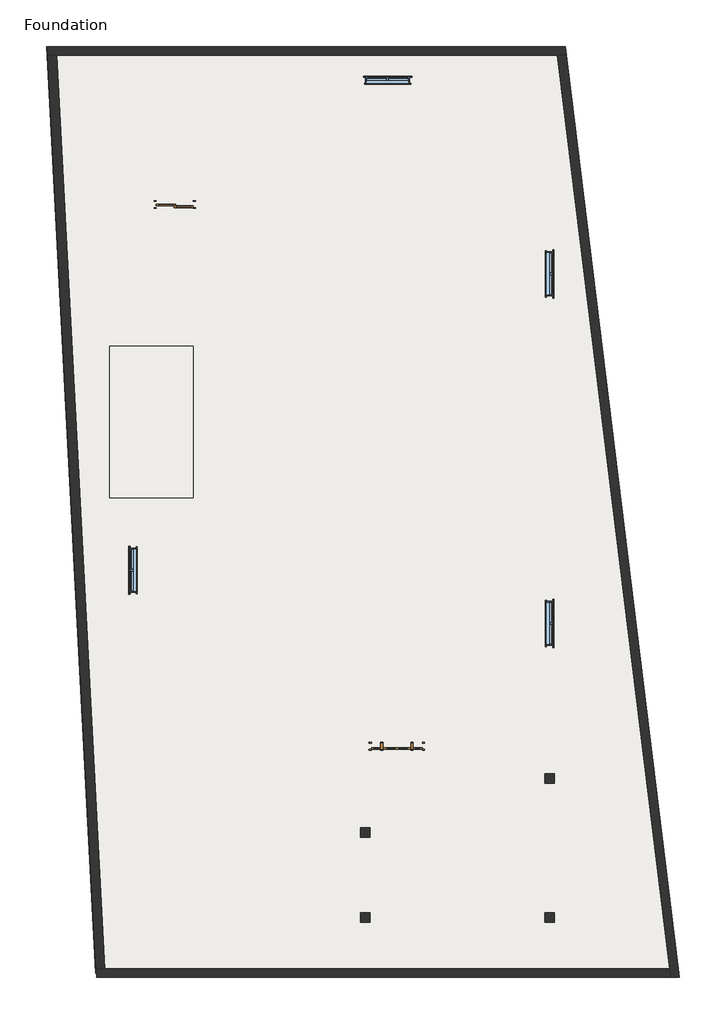
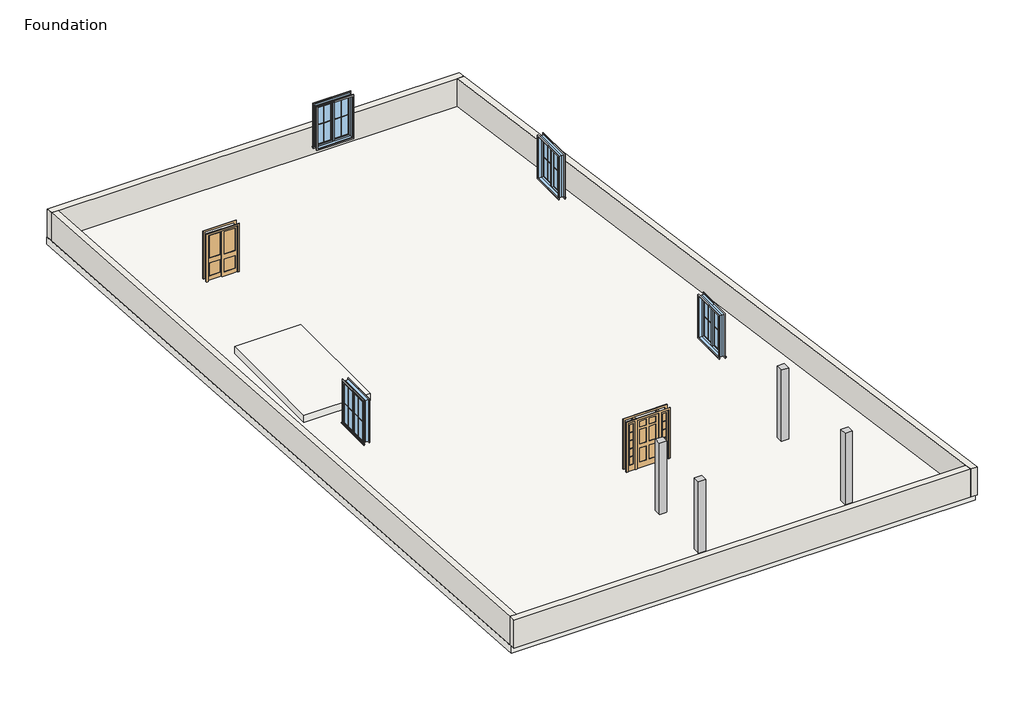
# One storey: 16 proxies, 4 columns, 4 walls, 4 windows, 2 doors, 2 slabs.
"""IFC4 building model written with IfcOpenShell, lengths in millimetres."""

import ifcopenshell
import ifcopenshell.guid

model = None  # the IFC model being written
_history = None  # IfcOwnerHistory: only IFC2X3 demands one
_inside = {}  # id of a spatial element -> (the spatial element, [elements in it])
_under = {}  # id of a project, library or spatial element -> (it, [spatial elements below it])
_declared = {}  # id of a project -> (the project, [libraries it declares])
_typed = {}  # id of a type object -> (the type object, [elements of that type])
_made_of = {}  # id of a material, layer set ... -> (it, [elements and type objects made of it])


def new_model(schema):
    """Start an empty IFC model of exactly this schema.

    Asked for "IFC4X3", IfcOpenShell would pick the latest addendum, in which some entities
    have other attributes; the version numbers below select the first issue.
    IFC2X3 requires an IfcOwnerHistory on every rooted entity: one is made here for all.
    """
    global model, _history
    if schema == "IFC4X3":
        model = ifcopenshell.file(schema_version=(4, 3, 0, 0))
    else:
        model = ifcopenshell.file(schema=schema)
    _inside.clear()
    _under.clear()
    _declared.clear()
    _typed.clear()
    _made_of.clear()
    _history = None
    if model.schema == "IFC2X3":
        org = make("IfcOrganization", Name="unknown")
        user = make(
            "IfcPersonAndOrganization",
            ThePerson=make("IfcPerson", FamilyName="unknown"),
            TheOrganization=org,
        )
        app = make(
            "IfcApplication",
            ApplicationDeveloper=org,
            Version="unknown",
            ApplicationFullName="unknown",
            ApplicationIdentifier="unknown",
        )
        _history = make(
            "IfcOwnerHistory",
            OwningUser=user,
            OwningApplication=app,
            ChangeAction="ADDED",
            CreationDate=0,
        )
    return model


def make(cls, **values):
    """One entity of the class cls with the attributes given. An attribute that is None is left unset."""
    return model.create_entity(
        cls, **{name: value for name, value in values.items() if value is not None}
    )


def rooted(cls, **values):
    """An entity with a GlobalId (a new one), such as an element, a storey or a relation."""
    return make(cls, GlobalId=ifcopenshell.guid.new(), OwnerHistory=_history, **values)


def si_unit(unit_type, name, prefix=None):
    """IfcSIUnit, for example si_unit("LENGTHUNIT", "METRE", prefix="MILLI")."""
    return make("IfcSIUnit", UnitType=unit_type, Prefix=prefix, Name=name)


def assignment(units):
    """IfcUnitAssignment: the units of a project."""
    return None if units is None else make("IfcUnitAssignment", Units=units)


def point(xyz):
    """IfcCartesianPoint."""
    return None if xyz is None else make("IfcCartesianPoint", Coordinates=xyz)


def direction(xyz):
    """IfcDirection."""
    return None if xyz is None else make("IfcDirection", DirectionRatios=xyz)


def frame(location, z_axis=None, x_axis=None):
    """IfcAxis2Placement3D, a coordinate frame: its origin and axes. An axis left out is left unset."""
    return make(
        "IfcAxis2Placement3D",
        Location=point(location),
        Axis=direction(z_axis),
        RefDirection=direction(x_axis),
    )


def origin():
    """The frame at (0, 0, 0) with its axes left unset."""
    return frame((0.0, 0.0, 0.0))


def origin_with_axes():
    """The frame at (0, 0, 0) with the z axis (0, 0, 1) and the x axis (1, 0, 0) written out."""
    return frame((0.0, 0.0, 0.0), z_axis=(0.0, 0.0, 1.0), x_axis=(1.0, 0.0, 0.0))


def place(relative_to, where):
    """IfcLocalPlacement: puts the frame where relative to a parent placement (None: the world)."""
    return make(
        "IfcLocalPlacement", PlacementRelTo=relative_to, RelativePlacement=where
    )


def context(
    kind, dimensions, precision=None, world=None, true_north=None, identifier=None
):
    """IfcGeometricRepresentationContext, for example the 3D "Model" context."""
    return make(
        "IfcGeometricRepresentationContext",
        ContextIdentifier=identifier,
        ContextType=kind,
        CoordinateSpaceDimension=dimensions,
        Precision=precision,
        WorldCoordinateSystem=world,
        TrueNorth=true_north,
    )


def project(units=None, contexts=None):
    """IfcProject with its units and contexts."""
    return rooted(
        "IfcProject",
        Name="project",
        RepresentationContexts=contexts,
        UnitsInContext=assignment(units),
    )


def spatial(cls, under=None, at=None, **own):
    """A site, building, storey or space (cls), placed at a placement, below another one or the project."""
    s = rooted(cls, ObjectPlacement=at, **own)
    if under is not None:
        _under.setdefault(under.id(), (under, []))[1].append(s)
    return s


def polyline(points):
    """IfcPolyline through the points."""
    return make("IfcPolyline", Points=[point(p) for p in points])


def outline(outer, holes=None, kind="AREA"):
    """IfcArbitraryClosedProfileDef: a profile drawn as a closed curve; with holes, ...WithVoids."""
    if holes is None:
        return make("IfcArbitraryClosedProfileDef", ProfileType=kind, OuterCurve=outer)
    return make(
        "IfcArbitraryProfileDefWithVoids",
        ProfileType=kind,
        OuterCurve=outer,
        InnerCurves=holes,
    )


def extrude(swept, where, along, depth):
    """IfcExtrudedAreaSolid: the profile swept, set in the frame where, extruded along a direction by depth."""
    return make(
        "IfcExtrudedAreaSolid",
        SweptArea=swept,
        Position=where,
        ExtrudedDirection=direction(along),
        Depth=depth,
    )


def faces_of(points, faces, orient=None, outer=None):
    """IfcFace entities. A face is a list of loops; a loop is a list of indices into points, from 0.

    orient and outer hold one flag for each loop. By default every Orientation is true, the
    first loop of a face is its IfcFaceOuterBound and the others are IfcFaceBound.
    """
    made = []
    for i, loops in enumerate(faces):
        bounds = []
        for j, loop in enumerate(loops):
            is_outer = j == 0 if outer is None else outer[i][j]
            bounds.append(
                make(
                    "IfcFaceOuterBound" if is_outer else "IfcFaceBound",
                    Bound=make("IfcPolyLoop", Polygon=[points[k] for k in loop]),
                    Orientation=True if orient is None else orient[i][j],
                )
            )
        made.append(make("IfcFace", Bounds=bounds))
    return made


def faceted_brep(points, faces, orient=None, outer=None, voids=None):
    """IfcFacetedBrep: a solid bounded by flat faces; with voids (closed shells), ...WithVoids."""
    shared = [point(p) for p in points]
    hull = make("IfcClosedShell", CfsFaces=faces_of(shared, faces, orient, outer))
    if voids is None:
        return make("IfcFacetedBrep", Outer=hull)
    return make(
        "IfcFacetedBrepWithVoids",
        Outer=hull,
        Voids=[
            make(cls, CfsFaces=faces_of(shared, fs, o, b)) for cls, fs, o, b in voids
        ],
    )


def shape(context_of_items, identifier, shape_type, items):
    """IfcShapeRepresentation: the items that make up one representation, for example the "Body"."""
    return make(
        "IfcShapeRepresentation",
        ContextOfItems=context_of_items,
        RepresentationIdentifier=identifier,
        RepresentationType=shape_type,
        Items=items,
    )


def source(mapping_origin, context_of_items, identifier, shape_type, items):
    """IfcRepresentationMap: a shape defined once, which mapped items show again and again."""
    return make(
        "IfcRepresentationMap",
        MappingOrigin=mapping_origin,
        MappedRepresentation=shape(context_of_items, identifier, shape_type, items),
    )


def transform(
    local_origin,
    x_axis=None,
    y_axis=None,
    z_axis=None,
    scale=None,
    scale2=None,
    scale3=None,
    uniform=True,
):
    """IfcCartesianTransformationOperator3D, or its non-uniform kind. x_axis, y_axis, z_axis: its Axis1, 2, 3."""
    if uniform:
        return make(
            "IfcCartesianTransformationOperator3D",
            Axis1=direction(x_axis),
            Axis2=direction(y_axis),
            LocalOrigin=point(local_origin),
            Scale=scale,
            Axis3=direction(z_axis),
        )
    return make(
        "IfcCartesianTransformationOperator3DnonUniform",
        Axis1=direction(x_axis),
        Axis2=direction(y_axis),
        LocalOrigin=point(local_origin),
        Scale=scale,
        Axis3=direction(z_axis),
        Scale2=scale2,
        Scale3=scale3,
    )


def mapped(mapping_source, mapping_target):
    """IfcMappedItem: shows the shape of a source again, moved by a transform."""
    return make(
        "IfcMappedItem", MappingSource=mapping_source, MappingTarget=mapping_target
    )


def made_of(thing, what):
    """Note that an element or type object is made of a material, layer set ...; save() writes the relation."""
    if what is not None:
        _made_of.setdefault(what.id(), (what, []))[1].append(thing)
    return thing


def element(
    cls,
    number,
    at=None,
    inside=None,
    cuts=None,
    type_object=None,
    material=None,
    context=None,
    identifier="Body",
    shape_type=None,
    held_by="IfcProductDefinitionShape",
    body=None,
    shapes=None,
    **own,
):
    """One element of the class cls, such as IfcWall. Its Tag is "e" and its number.

    at: its placement. inside: the storey or other place that contains it. cuts: it is an
    opening in that element (IfcRelVoidsElement). A single representation is given by context,
    identifier, shape_type and body (its items); several are given by shapes. held_by: the class
    of the entity that holds the representations. save() writes the other relations.
    """
    e = rooted(cls, Tag="e%d" % number, ObjectPlacement=at, **own)
    if body is not None:
        shapes = [shape(context, identifier, shape_type, body)]
    if shapes is not None:
        e.Representation = make(held_by, Representations=shapes)
    if inside is not None:
        _inside.setdefault(inside.id(), (inside, []))[1].append(e)
    if cuts is not None:
        rooted(
            "IfcRelVoidsElement", RelatingBuildingElement=cuts, RelatedOpeningElement=e
        )
    if type_object is not None:
        _typed.setdefault(type_object.id(), (type_object, []))[1].append(e)
    return made_of(e, material)


def aggregate(whole, parts):
    """IfcRelAggregates: a whole, such as a stair, and the parts it consists of."""
    return rooted("IfcRelAggregates", RelatingObject=whole, RelatedObjects=parts)


def save(model, path):
    """Write the relations noted so far, then the file.

    IfcRelAggregates (storeys below a building ...), IfcRelContainedInSpatialStructure (elements
    in a storey), IfcRelDefinesByType, IfcRelAssociatesMaterial and IfcRelDeclares: one each for
    every whole, place, type object, material and project.
    """
    for whole, parts in _under.values():
        aggregate(whole, parts)
    for where, things in _inside.values():
        rooted(
            "IfcRelContainedInSpatialStructure",
            RelatedElements=things,
            RelatingStructure=where,
        )
    for kind, things in _typed.values():
        rooted("IfcRelDefinesByType", RelatedObjects=things, RelatingType=kind)
    for what, things in _made_of.values():
        rooted("IfcRelAssociatesMaterial", RelatedObjects=things, RelatingMaterial=what)
    for by, libraries in _declared.values():
        rooted("IfcRelDeclares", RelatingContext=by, RelatedDefinitions=libraries)
    model.write(path)


def muntin_pattern_2x2_muntin_pattern_2x2_bff912c5(model_context):
    return source(origin(), model_context, "Body", "SweptSolid", [
        extrude(outline(polyline([(850.9, -6.35), (850.9, -293.6875), (838.2, -293.6875), (838.2, -6.35), (0.0, -6.35), (0.0, 6.35), (838.2, 6.35), (838.2, 293.6875), (850.9, 293.6875), (850.9, 6.35), (1689.1, 6.35), (1689.1, -6.35), (850.9, -6.35)])), frame((0.0, 9.525, 0.0), z_axis=(0.0, 1.0, 0.0), x_axis=(0.0, 0.0, 1.0)), (0.0, 0.0, 1.0), 12.7),
        extrude(outline(polyline([(850.9, -6.35), (850.9, -293.6875), (838.2, -293.6875), (838.2, -6.35), (0.0, -6.35), (0.0, 6.35), (838.2, 6.35), (838.2, 293.6875), (850.9, 293.6875), (850.9, 6.35), (1689.1, 6.35), (1689.1, -6.35), (850.9, -6.35)])), frame((0.0, -22.225, 0.0), z_axis=(0.0, 1.0, 0.0), x_axis=(0.0, 0.0, 1.0)), (0.0, 0.0, 1.0), 12.7),
    ])


def muntin_pattern_2x2_muntin_pattern_2x2_c2194282(model_context):
    return source(origin(), model_context, "Body", "SweptSolid", [
        extrude(outline(polyline([(850.9, -6.35), (850.9, -293.6875), (838.2, -293.6875), (838.2, -6.35), (0.0, -6.35), (0.0, 6.35), (838.2, 6.35), (838.2, 293.6875), (850.9, 293.6875), (850.9, 6.35), (1689.1, 6.35), (1689.1, -6.35), (850.9, -6.35)])), frame((0.0, -22.225, 0.0), z_axis=(0.0, 1.0, 0.0), x_axis=(0.0, 0.0, 1.0)), (0.0, 0.0, 1.0), 12.7),
        extrude(outline(polyline([(850.9, -6.35), (850.9, -293.6875), (838.2, -293.6875), (838.2, -6.35), (0.0, -6.35), (0.0, 6.35), (838.2, 6.35), (838.2, 293.6875), (850.9, 293.6875), (850.9, 6.35), (1689.1, 6.35), (1689.1, -6.35), (850.9, -6.35)])), frame((0.0, 9.525, 0.0), z_axis=(0.0, 1.0, 0.0), x_axis=(0.0, 0.0, 1.0)), (0.0, 0.0, 1.0), 12.7),
    ])


def trim_window_exterior_flat_with_sill_e04b3088(model_context):
    return source(origin(), model_context, "Body", "SweptSolid", [
        extrude(outline(polyline([(781.05, -1850.9823709), (781.05, -1908.1323709), (-781.05, -1908.1323709), (-781.05, -1850.9823709), (781.05, -1850.9823709)])), origin_with_axes(), (0.0, 0.0, 1.0), 19.05),
        extrude(outline(polyline([(-1860.55, 38.1), (-1831.2580645, 38.1), (-1828.8, 19.05), (-1828.8, 0.0), (-1850.9823709, 0.0), (-1850.9823709, 19.05), (-1860.55, 19.05), (-1860.55, 38.1)])), frame((-793.75, 0.0, 0.0), z_axis=(1.0, 0.0, 0.0), x_axis=(0.0, 1.0, 0.0)), (0.0, 0.0, 1.0), 1587.5),
        extrude(outline(polyline([(-781.05, 57.15), (781.05, 57.15), (781.05, -1828.8), (723.9, -1828.8), (723.9, 0.0), (-723.9, 0.0), (-723.9, -1828.8), (-781.05, -1828.8), (-781.05, 57.15)])), origin_with_axes(), (0.0, 0.0, 1.0), 19.05),
    ])


def trim_window_interior_flat_picture_frame_2a7685fe(model_context):
    return source(origin(), model_context, "Body", "SweptSolid", [
        extrude(outline(polyline([(768.35, 44.45), (768.35, -1873.25), (-768.35, -1873.25), (-768.35, 44.45), (768.35, 44.45)]), holes=[polyline([(711.2, -12.7), (-711.2, -12.7), (-711.2, -1816.1), (711.2, -1816.1), (711.2, -12.7)])]), origin_with_axes(), (0.0, 0.0, 1.0), 31.75),
    ])


def column_96c5ed10(model_context):
    return source(origin(), model_context, "Body", "SweptSolid", [
        extrude(outline(polyline([(152.4, 152.4), (152.4, -152.4), (-152.4, -152.4), (-152.4, 152.4), (152.4, 152.4)])), frame((0.0, 0.0, -381.0), z_axis=(0.0, 0.0, 1.0), x_axis=(1.0, 0.0, 0.0)), (0.0, 0.0, 1.0), 3124.2),
    ])


def door_4cad2e7a(model_context):
    return source(origin(), model_context, "Body", "SweptSolid", [
        extrude(outline(polyline([(762.0, 60.325), (609.6, 60.325), (609.6, 92.075), (762.0, 92.075), (762.0, 60.325)])), frame((0.0, 0.0, 600.075), z_axis=(0.0, 0.0, 1.0), x_axis=(1.0, 0.0, 0.0)), (0.0, 0.0, 1.0), 19.05),
        extrude(outline(polyline([(762.0, 60.325), (609.6, 60.325), (609.6, 92.075), (762.0, 92.075), (762.0, 60.325)])), frame((0.0, 0.0, 955.675), z_axis=(0.0, 0.0, 1.0), x_axis=(1.0, 0.0, 0.0)), (0.0, 0.0, 1.0), 19.05),
        extrude(outline(polyline([(762.0, 60.325), (609.6, 60.325), (609.6, 92.075), (762.0, 92.075), (762.0, 60.325)])), frame((0.0, 0.0, 1311.275), z_axis=(0.0, 0.0, 1.0), x_axis=(1.0, 0.0, 0.0)), (0.0, 0.0, 1.0), 19.05),
        extrude(outline(polyline([(762.0, 60.325), (609.6, 60.325), (609.6, 92.075), (762.0, 92.075), (762.0, 60.325)])), frame((0.0, 0.0, 1666.875), z_axis=(0.0, 0.0, 1.0), x_axis=(1.0, 0.0, 0.0)), (0.0, 0.0, 1.0), 19.05),
        extrude(outline(polyline([(-609.6, 60.325), (-762.0, 60.325), (-762.0, 92.075), (-609.6, 92.075), (-609.6, 60.325)])), frame((0.0, 0.0, 1666.875), z_axis=(0.0, 0.0, 1.0), x_axis=(1.0, 0.0, 0.0)), (0.0, 0.0, 1.0), 19.05),
        extrude(outline(polyline([(-609.6, 60.325), (-762.0, 60.325), (-762.0, 92.075), (-609.6, 92.075), (-609.6, 60.325)])), frame((0.0, 0.0, 1311.275), z_axis=(0.0, 0.0, 1.0), x_axis=(1.0, 0.0, 0.0)), (0.0, 0.0, 1.0), 19.05),
        extrude(outline(polyline([(-609.6, 60.325), (-762.0, 60.325), (-762.0, 92.075), (-609.6, 92.075), (-609.6, 60.325)])), frame((0.0, 0.0, 955.675), z_axis=(0.0, 0.0, 1.0), x_axis=(1.0, 0.0, 0.0)), (0.0, 0.0, 1.0), 19.05),
        extrude(outline(polyline([(-609.6, 60.325), (-762.0, 60.325), (-762.0, 92.075), (-609.6, 92.075), (-609.6, 60.325)])), frame((0.0, 0.0, 600.075), z_axis=(0.0, 0.0, 1.0), x_axis=(1.0, 0.0, 0.0)), (0.0, 0.0, 1.0), 19.05),
        extrude(outline(polyline([(762.0, 66.675), (609.6, 66.675), (609.6, 85.725), (762.0, 85.725), (762.0, 66.675)])), frame((0.0, 0.0, 254.0), z_axis=(0.0, 0.0, 1.0), x_axis=(1.0, 0.0, 0.0)), (0.0, 0.0, 1.0), 1778.0),
        extrude(outline(polyline([(-609.6, 66.675), (-762.0, 66.675), (-762.0, 85.725), (-609.6, 85.725), (-609.6, 66.675)])), frame((0.0, 0.0, 254.0), z_axis=(0.0, 0.0, 1.0), x_axis=(1.0, 0.0, 0.0)), (0.0, 0.0, 1.0), 1778.0),
        extrude(outline(polyline([(-457.2, -101.6), (-533.4, -101.6), (-533.4, 101.6), (-457.2, 101.6), (-457.2, -101.6)])), origin_with_axes(), (0.0, 0.0, 1.0), 2133.6),
        extrude(outline(polyline([(533.4, -101.6), (457.2, -101.6), (457.2, 101.6), (533.4, 101.6), (533.4, -101.6)])), origin_with_axes(), (0.0, 0.0, 1.0), 2133.6),
        extrude(outline(polyline([(2133.6, -533.4), (2133.6, -838.2), (0.0, -838.2), (0.0, -533.4), (2133.6, -533.4)]), holes=[polyline([(2032.0, -609.6), (254.0, -609.6), (254.0, -762.0), (2032.0, -762.0), (2032.0, -609.6)])]), frame((0.0, 50.8, 0.0), z_axis=(0.0, 1.0, 0.0), x_axis=(0.0, 0.0, 1.0)), (0.0, 0.0, 1.0), 50.8),
        extrude(outline(polyline([(0.0, 533.4), (0.0, 838.2), (2133.6, 838.2), (2133.6, 533.4), (0.0, 533.4)]), holes=[polyline([(2032.0, 762.0), (254.0, 762.0), (254.0, 609.6), (2032.0, 609.6), (2032.0, 762.0)])]), frame((0.0, 50.8, 0.0), z_axis=(0.0, 1.0, 0.0), x_axis=(0.0, 0.0, 1.0)), (0.0, 0.0, 1.0), 50.8),
        extrude(outline(polyline([(0.0, -914.4), (0.0, -838.2), (2133.6, -838.2), (2133.6, -533.4), (0.0, -533.4), (0.0, -457.2), (2133.6, -457.2), (2133.6, 457.2), (0.0, 457.2), (0.0, 533.4), (2133.6, 533.4), (2133.6, 838.2), (0.0, 838.2), (0.0, 914.4), (2209.8, 914.4), (2209.8, -914.4), (0.0, -914.4)])), frame((0.0, -127.0, 0.0), z_axis=(0.0, 1.0, 0.0), x_axis=(0.0, 0.0, 1.0)), (0.0, 0.0, 1.0), 25.4),
        extrude(outline(polyline([(0.0, 914.4), (2209.8, 914.4), (2209.8, -914.4), (0.0, -914.4), (0.0, -838.2), (2133.6, -838.2), (2133.6, -533.4), (0.0, -533.4), (0.0, -457.2), (2133.6, -457.2), (2133.6, 457.2), (0.0, 457.2), (0.0, 533.4), (2133.6, 533.4), (2133.6, 838.2), (0.0, 838.2), (0.0, 914.4)])), frame((0.0, 101.6, 0.0), z_axis=(0.0, 1.0, 0.0), x_axis=(0.0, 0.0, 1.0)), (0.0, 0.0, 1.0), 25.4),
        extrude(outline(polyline([(-63.5, 63.5), (-330.2, 63.5), (-330.2, 88.9), (-63.5, 88.9), (-63.5, 63.5)])), frame((0.0, 0.0, 1778.0), z_axis=(0.0, 0.0, 1.0), x_axis=(1.0, 0.0, 0.0)), (0.0, 0.0, 1.0), 254.0),
        extrude(outline(polyline([(330.2, 63.5), (63.5, 63.5), (63.5, 88.9), (330.2, 88.9), (330.2, 63.5)])), frame((0.0, 0.0, 1778.0), z_axis=(0.0, 0.0, 1.0), x_axis=(1.0, 0.0, 0.0)), (0.0, 0.0, 1.0), 254.0),
        extrude(outline(polyline([(-63.5, 63.5), (-330.2, 63.5), (-330.2, 88.9), (-63.5, 88.9), (-63.5, 63.5)])), frame((0.0, 0.0, 1041.4), z_axis=(0.0, 0.0, 1.0), x_axis=(1.0, 0.0, 0.0)), (0.0, 0.0, 1.0), 635.0),
        extrude(outline(polyline([(330.2, 63.5), (63.5, 63.5), (63.5, 88.9), (330.2, 88.9), (330.2, 63.5)])), frame((0.0, 0.0, 1041.4), z_axis=(0.0, 0.0, 1.0), x_axis=(1.0, 0.0, 0.0)), (0.0, 0.0, 1.0), 635.0),
        extrude(outline(polyline([(-63.5, 63.5), (-330.2, 63.5), (-330.2, 88.9), (-63.5, 88.9), (-63.5, 63.5)])), frame((0.0, 0.0, 254.0), z_axis=(0.0, 0.0, 1.0), x_axis=(1.0, 0.0, 0.0)), (0.0, 0.0, 1.0), 609.6),
        extrude(outline(polyline([(330.2, 63.5), (63.5, 63.5), (63.5, 88.9), (330.2, 88.9), (330.2, 63.5)])), frame((0.0, 0.0, 254.0), z_axis=(0.0, 0.0, 1.0), x_axis=(1.0, 0.0, 0.0)), (0.0, 0.0, 1.0), 609.6),
        extrude(outline(polyline([(2133.6, 457.2), (2133.6, -457.2), (0.0, -457.2), (0.0, 457.2), (2133.6, 457.2)]), holes=[polyline([(2032.0, -63.5), (1778.0, -63.5), (1778.0, -330.2), (2032.0, -330.2), (2032.0, -63.5)]), polyline([(2032.0, 330.2), (1778.0, 330.2), (1778.0, 63.5), (2032.0, 63.5), (2032.0, 330.2)]), polyline([(1676.4, -63.5), (1041.4, -63.5), (1041.4, -330.2), (1676.4, -330.2), (1676.4, -63.5)]), polyline([(1676.4, 330.2), (1041.4, 330.2), (1041.4, 63.5), (1676.4, 63.5), (1676.4, 330.2)]), polyline([(863.6, -63.5), (254.0, -63.5), (254.0, -330.2), (863.6, -330.2), (863.6, -63.5)]), polyline([(863.6, 330.2), (254.0, 330.2), (254.0, 63.5), (863.6, 63.5), (863.6, 330.2)])]), frame((0.0, 50.8, 0.0), z_axis=(0.0, 1.0, 0.0), x_axis=(0.0, 0.0, 1.0)), (0.0, 0.0, 1.0), 50.8),
    ])


def door_5d877b8f(model_context):
    return source(origin(), model_context, "Body", "SweptSolid", [
        extrude(outline(polyline([(-63.5, 190.5), (-520.7, 190.5), (-520.7, 215.9), (-63.5, 215.9), (-63.5, 190.5)])), frame((0.0, 0.0, 965.2), z_axis=(0.0, 0.0, 1.0), x_axis=(1.0, 0.0, 0.0)), (0.0, 0.0, 1.0), 977.9),
        extrude(outline(polyline([(-63.5, 190.5), (-520.7, 190.5), (-520.7, 215.9), (-63.5, 215.9), (-63.5, 190.5)])), frame((0.0, 0.0, 184.15), z_axis=(0.0, 0.0, 1.0), x_axis=(1.0, 0.0, 0.0)), (0.0, 0.0, 1.0), 565.15),
        extrude(outline(polyline([(63.5, 165.1), (520.7, 165.1), (520.7, 139.7), (63.5, 139.7), (63.5, 165.1)])), frame((0.0, 0.0, 965.2), z_axis=(0.0, 0.0, 1.0), x_axis=(1.0, 0.0, 0.0)), (0.0, 0.0, 1.0), 977.9),
        extrude(outline(polyline([(63.5, 165.1), (520.7, 165.1), (520.7, 139.7), (63.5, 139.7), (63.5, 165.1)])), frame((0.0, 0.0, 184.15), z_axis=(0.0, 0.0, 1.0), x_axis=(1.0, 0.0, 0.0)), (0.0, 0.0, 1.0), 565.15),
        extrude(outline(polyline([(2032.0, 25.4), (2032.0, -609.6), (0.0, -609.6), (0.0, 25.4), (2032.0, 25.4)]), holes=[polyline([(184.15, -520.7), (749.3, -520.7), (749.3, -63.5), (184.15, -63.5), (184.15, -520.7)]), polyline([(965.2, -520.7), (1943.1, -520.7), (1943.1, -63.5), (965.2, -63.5), (965.2, -520.7)])]), frame((0.0, 177.8, 0.0), z_axis=(0.0, 1.0, 0.0), x_axis=(0.0, 0.0, 1.0)), (0.0, 0.0, 1.0), 50.8),
        extrude(outline(polyline([(0.0, -685.8), (0.0, -609.6), (2032.0, -609.6), (2032.0, 609.6), (0.0, 609.6), (0.0, 685.8), (2108.2, 685.8), (2108.2, -685.8), (0.0, -685.8)])), frame((0.0, 0.0, 0.0), z_axis=(0.0, 1.0, 0.0), x_axis=(0.0, 0.0, 1.0)), (0.0, 0.0, 1.0), 25.4),
        extrude(outline(polyline([(0.0, 685.8), (2108.2, 685.8), (2108.2, -685.8), (0.0, -685.8), (0.0, -609.6), (2032.0, -609.6), (2032.0, 609.6), (0.0, 609.6), (0.0, 685.8)])), frame((0.0, 228.6, 0.0), z_axis=(0.0, 1.0, 0.0), x_axis=(0.0, 0.0, 1.0)), (0.0, 0.0, 1.0), 25.4),
        extrude(outline(polyline([(2032.0, -25.4), (0.0, -25.4), (0.0, 609.6), (2032.0, 609.6), (2032.0, -25.4)]), holes=[polyline([(965.2, 520.7), (965.2, 63.5), (1943.1, 63.5), (1943.1, 520.7), (965.2, 520.7)]), polyline([(184.15, 520.7), (184.15, 63.5), (749.3, 63.5), (749.3, 520.7), (184.15, 520.7)])]), frame((0.0, 127.0, 0.0), z_axis=(0.0, 1.0, 0.0), x_axis=(0.0, 0.0, 1.0)), (0.0, 0.0, 1.0), 50.8),
    ])


def window_c580ef63(model_context):
    return source(origin(), model_context, "Body", "SolidModel", [
        faceted_brep([(9.525, 120.65, 2730.5), (-9.525, 120.65, 2730.5), (-9.525, 69.85, 2730.5), (9.525, 69.85, 2730.5), (9.525, 120.65, 927.1), (9.525, 69.85, 927.1), (-9.525, 69.85, 927.1), (-9.525, 120.65, 927.1), (-9.525, 69.85, 946.15), (-9.525, 69.85, 2711.45), (-30.1625, 69.85, 946.15), (-30.1625, 69.85, 2711.45), (-30.1625, 6.35, 946.15), (-30.1625, 6.35, 2711.45), (30.1625, 6.35, 946.15), (30.1625, 6.35, 2711.45), (30.1625, 69.85, 946.15), (30.1625, 69.85, 2711.45), (9.525, 69.85, 946.15), (9.525, 69.85, 2711.45)], [[[0, 1, 2, 3]], [[4, 5, 6, 7]], [[1, 0, 4, 7]], [[2, 1, 7, 6, 8, 9]], [[9, 8, 10, 11]], [[11, 10, 12, 13]], [[13, 12, 14, 15]], [[15, 14, 16, 17]], [[17, 16, 18, 19]], [[0, 3, 19, 18, 5, 4]], [[18, 8, 6, 5]], [[9, 19, 3, 2]], [[8, 18, 16, 14, 12, 10]], [[19, 9, 11, 13, 15, 17]]]),
        extrude(outline(polyline([(-66.675, 101.6), (-66.675, 95.25), (-654.05, 95.25), (-654.05, 101.6), (-66.675, 101.6)])), frame((0.0, 0.0, 984.25), z_axis=(0.0, 0.0, 1.0), x_axis=(1.0, 0.0, 0.0)), (0.0, 0.0, 1.0), 1689.1),
        extrude(outline(polyline([(-654.05, 82.55), (-654.05, 88.9), (-66.675, 88.9), (-66.675, 82.55), (-654.05, 82.55)])), frame((0.0, 0.0, 984.25), z_axis=(0.0, 0.0, 1.0), x_axis=(1.0, 0.0, 0.0)), (0.0, 0.0, 1.0), 1689.1),
        extrude(outline(polyline([(654.05, 101.6), (654.05, 95.25), (66.675, 95.25), (66.675, 101.6), (654.05, 101.6)])), frame((0.0, 0.0, 984.25), z_axis=(0.0, 0.0, 1.0), x_axis=(1.0, 0.0, 0.0)), (0.0, 0.0, 1.0), 1689.1),
        extrude(outline(polyline([(66.675, 82.55), (66.675, 88.9), (654.05, 88.9), (654.05, 82.55), (66.675, 82.55)])), frame((0.0, 0.0, 984.25), z_axis=(0.0, 0.0, 1.0), x_axis=(1.0, 0.0, 0.0)), (0.0, 0.0, 1.0), 1689.1),
        extrude(outline(polyline([(2730.5, -711.2), (927.1, -711.2), (927.1, -9.525), (2730.5, -9.525), (2730.5, -711.2)]), holes=[polyline([(2673.35, -66.675), (984.25, -66.675), (984.25, -654.05), (2673.35, -654.05), (2673.35, -66.675)])]), frame((0.0, 69.85, 0.0), z_axis=(0.0, 1.0, 0.0), x_axis=(0.0, 0.0, 1.0)), (0.0, 0.0, 1.0), 44.45),
        extrude(outline(polyline([(927.1, 711.2), (2730.5, 711.2), (2730.5, 9.525), (927.1, 9.525), (927.1, 711.2)]), holes=[polyline([(984.25, 66.675), (2673.35, 66.675), (2673.35, 654.05), (984.25, 654.05), (984.25, 66.675)])]), frame((0.0, 69.85, 0.0), z_axis=(0.0, 1.0, 0.0), x_axis=(0.0, 0.0, 1.0)), (0.0, 0.0, 1.0), 44.45),
        extrude(outline(polyline([(2743.2, -723.9), (914.4, -723.9), (914.4, 723.9), (2743.2, 723.9), (2743.2, -723.9)]), holes=[polyline([(2724.15, 704.85), (933.45, 704.85), (933.45, -704.85), (2724.15, -704.85), (2724.15, 704.85)])]), frame((0.0, -101.6, 0.0), z_axis=(0.0, 1.0, 0.0), x_axis=(0.0, 0.0, 1.0)), (0.0, 0.0, 1.0), 107.95),
        faceted_brep([(692.15, 69.85, 2711.45), (692.15, 6.35, 2711.45), (-692.15, 6.35, 2711.45), (-692.15, 69.85, 2711.45), (711.2, 120.65, 2730.5), (711.2, 69.85, 2730.5), (-711.2, 69.85, 2730.5), (-711.2, 120.65, 2730.5), (723.9, 6.35, 2743.2), (723.9, 120.65, 2743.2), (-723.9, 120.65, 2743.2), (-723.9, 6.35, 2743.2), (-692.15, 6.35, 946.15), (-692.15, 69.85, 946.15), (-711.2, 69.85, 927.1), (-711.2, 120.65, 927.1), (-723.9, 120.65, 914.4), (-723.9, 6.35, 914.4), (692.15, 6.35, 946.15), (692.15, 69.85, 946.15), (711.2, 69.85, 927.1), (711.2, 120.65, 927.1), (723.9, 120.65, 914.4), (723.9, 6.35, 914.4)], [[[0, 1, 2, 3]], [[4, 5, 6, 7]], [[8, 9, 10, 11]], [[3, 2, 12, 13]], [[7, 6, 14, 15]], [[11, 10, 16, 17]], [[13, 12, 18, 19]], [[15, 14, 20, 21]], [[17, 16, 22, 23]], [[11, 17, 23, 8], [1, 18, 12, 2]], [[19, 18, 1, 0]], [[5, 20, 14, 6], [3, 13, 19, 0]], [[21, 20, 5, 4]], [[23, 22, 9, 8]], [[9, 22, 16, 10], [7, 15, 21, 4]]]),
    ])


model = new_model("IFC4")

# Units and contexts
model_context = context("Model", 3, world=origin())
ifc_project = project(units=[si_unit("LENGTHUNIT", "METRE", prefix="MILLI")], contexts=[model_context])

# Site, building, storey
site = spatial("IfcSite", under=ifc_project)
building = spatial("IfcBuilding", under=site)
storey = spatial("IfcBuildingStorey", under=building, Name="Foundation", Elevation=-381.0)

# Proxies
placement = place(None, origin())
muntin_pattern_2x2_muntin_pattern_2x2_shape = muntin_pattern_2x2_muntin_pattern_2x2_bff912c5(model_context)
element("IfcBuildingElementProxy", 1, Name="Muntin Pattern_2x2 : Muntin Pattern_2x2", ObjectType="Muntin Pattern_2x2 : Muntin Pattern_2x2", at=placement, inside=storey, context=model_context, shape_type="MappedRepresentation", body=[
    mapped(muntin_pattern_2x2_muntin_pattern_2x2_shape, transform((-4271.6763913, -8364.6154211, 603.25), x_axis=(0.0, 1.0, 0.0), y_axis=(-1.0, 0.0, 0.0), z_axis=(0.0, 0.0, 1.0))),
])
element("IfcBuildingElementProxy", 2, Name="Muntin Pattern_2x2 : Muntin Pattern_2x2", ObjectType="Muntin Pattern_2x2 : Muntin Pattern_2x2", at=placement, inside=storey, context=model_context, shape_type="MappedRepresentation", body=[
    mapped(muntin_pattern_2x2_muntin_pattern_2x2_shape, transform((9628.4736087, -9396.4904211, 603.25), x_axis=(0.0, -1.0, 0.0), y_axis=(1.0, 0.0, 0.0), z_axis=(0.0, 0.0, 1.0))),
])
element("IfcBuildingElementProxy", 3, Name="Muntin Pattern_2x2 : Muntin Pattern_2x2", ObjectType="Muntin Pattern_2x2 : Muntin Pattern_2x2", at=placement, inside=storey, context=model_context, shape_type="MappedRepresentation", body=[
    mapped(muntin_pattern_2x2_muntin_pattern_2x2_shape, transform((9628.4736087, 2109.7095789, 603.25), x_axis=(0.0, -1.0, 0.0), y_axis=(1.0, 0.0, 0.0), z_axis=(0.0, 0.0, 1.0))),
])
element("IfcBuildingElementProxy", 4, Name="Muntin Pattern_2x2 : Muntin Pattern_2x2", ObjectType="Muntin Pattern_2x2 : Muntin Pattern_2x2", at=placement, inside=storey, context=model_context, shape_type="MappedRepresentation", body=[
    mapped(muntin_pattern_2x2_muntin_pattern_2x2_shape, transform((3842.0361087, 8211.5138811, 603.25), x_axis=(1.0, 0.0, 0.0), y_axis=(0.0, 1.0, 0.0), z_axis=(0.0, 0.0, 1.0))),
])
muntin_pattern_2x2_muntin_pattern_2x2_2_shape = muntin_pattern_2x2_muntin_pattern_2x2_c2194282(model_context)
element("IfcBuildingElementProxy", 5, Name="Muntin Pattern_2x2 : Muntin Pattern_2x2", ObjectType="Muntin Pattern_2x2 : Muntin Pattern_2x2", at=placement, inside=storey, context=model_context, shape_type="MappedRepresentation", body=[
    mapped(muntin_pattern_2x2_muntin_pattern_2x2_2_shape, transform((-4271.6763913, -7643.8904211, 603.25), x_axis=(0.0, -1.0, 0.0), y_axis=(1.0, 0.0, 0.0), z_axis=(0.0, 0.0, 1.0))),
])
element("IfcBuildingElementProxy", 6, Name="Muntin Pattern_2x2 : Muntin Pattern_2x2", ObjectType="Muntin Pattern_2x2 : Muntin Pattern_2x2", at=placement, inside=storey, context=model_context, shape_type="MappedRepresentation", body=[
    mapped(muntin_pattern_2x2_muntin_pattern_2x2_2_shape, transform((9628.4736087, -10117.2154211, 603.25), x_axis=(0.0, 1.0, 0.0), y_axis=(-1.0, 0.0, 0.0), z_axis=(0.0, 0.0, 1.0))),
])
element("IfcBuildingElementProxy", 7, Name="Muntin Pattern_2x2 : Muntin Pattern_2x2", ObjectType="Muntin Pattern_2x2 : Muntin Pattern_2x2", at=placement, inside=storey, context=model_context, shape_type="MappedRepresentation", body=[
    mapped(muntin_pattern_2x2_muntin_pattern_2x2_2_shape, transform((9628.4736087, 1388.9845789, 603.25), x_axis=(0.0, 1.0, 0.0), y_axis=(-1.0, 0.0, 0.0), z_axis=(0.0, 0.0, 1.0))),
])
element("IfcBuildingElementProxy", 8, Name="Muntin Pattern_2x2 : Muntin Pattern_2x2", ObjectType="Muntin Pattern_2x2 : Muntin Pattern_2x2", at=placement, inside=storey, context=model_context, shape_type="MappedRepresentation", body=[
    mapped(muntin_pattern_2x2_muntin_pattern_2x2_2_shape, transform((4562.7611087, 8211.5138811, 603.25), x_axis=(-1.0, 0.0, 0.0), y_axis=(0.0, -1.0, 0.0), z_axis=(0.0, 0.0, 1.0))),
])
trim_window_exterior_flat_with_sill_shape = trim_window_exterior_flat_with_sill_e04b3088(model_context)
element("IfcBuildingElementProxy", 9, Name="Trim-Window-Exterior-Flat : with Sill", ObjectType="Trim-Window-Exterior-Flat : with Sill", at=placement, inside=storey, context=model_context, shape_type="MappedRepresentation", body=[
    mapped(trim_window_exterior_flat_with_sill_shape, transform((-4281.2013913, -8004.2529211, 2362.2), x_axis=(0.0, -1.0, 0.0), y_axis=(0.0, 0.0, 1.0), z_axis=(-1.0, 0.0, 0.0))),
])
element("IfcBuildingElementProxy", 10, Name="Trim-Window-Exterior-Flat : with Sill", ObjectType="Trim-Window-Exterior-Flat : with Sill", at=placement, inside=storey, context=model_context, shape_type="MappedRepresentation", body=[
    mapped(trim_window_exterior_flat_with_sill_shape, transform((9637.9986087, -9756.8529211, 2362.2), x_axis=(0.0, 1.0, 0.0), y_axis=(0.0, 0.0, 1.0), z_axis=(1.0, 0.0, 0.0))),
])
element("IfcBuildingElementProxy", 11, Name="Trim-Window-Exterior-Flat : with Sill", ObjectType="Trim-Window-Exterior-Flat : with Sill", at=placement, inside=storey, context=model_context, shape_type="MappedRepresentation", body=[
    mapped(trim_window_exterior_flat_with_sill_shape, transform((9637.9986087, 1749.3470789, 2362.2), x_axis=(0.0, 1.0, 0.0), y_axis=(0.0, 0.0, 1.0), z_axis=(1.0, 0.0, 0.0))),
])
element("IfcBuildingElementProxy", 12, Name="Trim-Window-Exterior-Flat : with Sill", ObjectType="Trim-Window-Exterior-Flat : with Sill", at=placement, inside=storey, context=model_context, shape_type="MappedRepresentation", body=[
    mapped(trim_window_exterior_flat_with_sill_shape, transform((4202.3986087, 8221.0388811, 2362.2), x_axis=(-1.0, 0.0, 0.0), y_axis=(0.0, 0.0, 1.0), z_axis=(0.0, 1.0, 0.0))),
])
trim_window_interior_flat_picture_frame_shape = trim_window_interior_flat_picture_frame_2a7685fe(model_context)
element("IfcBuildingElementProxy", 13, Name="Trim-Window-Interior-Flat : Picture Frame", ObjectType="Trim-Window-Interior-Flat : Picture Frame", at=placement, inside=storey, context=model_context, shape_type="MappedRepresentation", body=[
    mapped(trim_window_interior_flat_picture_frame_shape, transform((-4078.0013913, -8004.2529211, 2362.2), x_axis=(0.0, 1.0, 0.0), y_axis=(0.0, 0.0, 1.0), z_axis=(1.0, 0.0, 0.0))),
])
element("IfcBuildingElementProxy", 14, Name="Trim-Window-Interior-Flat : Picture Frame", ObjectType="Trim-Window-Interior-Flat : Picture Frame", at=placement, inside=storey, context=model_context, shape_type="MappedRepresentation", body=[
    mapped(trim_window_interior_flat_picture_frame_shape, transform((9434.7986087, -9756.8529211, 2362.2), x_axis=(0.0, -1.0, 0.0), y_axis=(0.0, 0.0, 1.0), z_axis=(-1.0, 0.0, 0.0))),
])
element("IfcBuildingElementProxy", 15, Name="Trim-Window-Interior-Flat : Picture Frame", ObjectType="Trim-Window-Interior-Flat : Picture Frame", at=placement, inside=storey, context=model_context, shape_type="MappedRepresentation", body=[
    mapped(trim_window_interior_flat_picture_frame_shape, transform((9434.7986087, 1749.3470789, 2362.2), x_axis=(0.0, -1.0, 0.0), y_axis=(0.0, 0.0, 1.0), z_axis=(-1.0, 0.0, 0.0))),
])
element("IfcBuildingElementProxy", 16, Name="Trim-Window-Interior-Flat : Picture Frame", ObjectType="Trim-Window-Interior-Flat : Picture Frame", at=placement, inside=storey, context=model_context, shape_type="MappedRepresentation", body=[
    mapped(trim_window_interior_flat_picture_frame_shape, transform((4202.3986087, 8017.8388811, 2362.2), x_axis=(1.0, 0.0, 0.0), y_axis=(0.0, 0.0, 1.0), z_axis=(0.0, -1.0, 0.0))),
])

# Columns
column_shape = column_96c5ed10(model_context)
element("IfcColumn", 17, ObjectType="Rectangular Column : 12\" x 12\"", at=placement, inside=storey, context=model_context, shape_type="MappedRepresentation", body=[
    mapped(column_shape, transform((3465.7986087, -16640.2529211, 0.0), x_axis=(0.0, 1.0, 0.0), y_axis=(-1.0, 0.0, 0.0), z_axis=(0.0, 0.0, 1.0))),
])
element("IfcColumn", 18, ObjectType="Rectangular Column : 12\" x 12\"", at=placement, inside=storey, context=model_context, shape_type="MappedRepresentation", body=[
    mapped(column_shape, transform((9536.3986087, -14862.2529211, 0.0), x_axis=(0.0, 1.0, 0.0), y_axis=(-1.0, 0.0, 0.0), z_axis=(0.0, 0.0, 1.0))),
])
element("IfcColumn", 19, ObjectType="Rectangular Column : 12\" x 12\"", at=placement, inside=storey, context=model_context, shape_type="MappedRepresentation", body=[
    mapped(column_shape, transform((9536.3986087, -19434.2529211, 0.0), x_axis=(0.0, 1.0, 0.0), y_axis=(-1.0, 0.0, 0.0), z_axis=(0.0, 0.0, 1.0))),
])
element("IfcColumn", 20, ObjectType="Rectangular Column : 12\" x 12\"", at=placement, inside=storey, context=model_context, shape_type="MappedRepresentation", body=[
    mapped(column_shape, transform((3465.7986087, -19434.2529211, 0.0), x_axis=(0.0, 1.0, 0.0), y_axis=(-1.0, 0.0, 0.0), z_axis=(0.0, 0.0, 1.0))),
])

# Doors
door_shape = door_4cad2e7a(model_context)
element("IfcDoor", 21, ObjectType="Single-Raised Panel with Sidelights : 36\" x 84\"", at=placement, inside=storey, context=model_context, shape_type="MappedRepresentation", body=[
    mapped(door_shape, transform((4507.1986087, -13795.4529211, -381.0), x_axis=(-1.0, 0.0, 0.0), y_axis=(0.0, -1.0, 0.0), z_axis=(0.0, 0.0, 1.0))),
])
door_2_shape = door_5d877b8f(model_context)
element("IfcDoor", 22, ObjectType="Sliding-Closet : 48\" x 80\"", at=placement, inside=storey, context=model_context, shape_type="MappedRepresentation", body=[
    mapped(door_2_shape, transform((-2808.0013913, 4162.3470789, -381.0), x_axis=(-1.0, 0.0, 0.0), y_axis=(0.0, -1.0, 0.0), z_axis=(0.0, 0.0, 1.0))),
])

# Slabs
element("IfcSlab", 23, ObjectType="Concrete Slab - 12\" 2", at=placement, inside=storey, context=model_context, shape_type="SweptSolid", body=[
    extrude(outline(polyline([(10025.1414378, 9232.4757765), (13795.4376886, -21276.6158374), (-5406.9623114, -21276.6158374), (-7033.0961859, 9232.4757765), (10025.1414378, 9232.4757765)])), frame((0.0, 0.0, -685.8), z_axis=(0.0, 0.0, 1.0), x_axis=(1.0, 0.0, 0.0)), (0.0, 0.0, 1.0), 304.8),
])
element("IfcSlab", 24, ObjectType="Generic - 12\" Grass", at=placement, inside=storey, context=model_context, shape_type="SweptSolid", body=[
    extrude(outline(polyline([(-4949.7178966, -638.2529211), (-2206.5178966, -638.2529211), (-2206.5178966, -5616.6529211), (-4949.7178966, -5616.6529211), (-4949.7178966, -638.2529211)])), frame((0.0, 0.0, -228.6), z_axis=(0.0, 0.0, 1.0), x_axis=(1.0, 0.0, 0.0)), (0.0, 0.0, 1.0), 304.8),
])

# Walls
element("IfcWall", 25, ObjectType="Exterior - Brick on Wood Stud", at=placement, inside=storey, context=model_context, shape_type="Brep", body=[
    faceted_brep([(-6987.4030616, 8949.9007765, -381.0), (-6704.4321039, 8949.9007765, -381.0), (9799.3910296, 8949.9007765, -381.0), (10084.0881186, 8949.9007765, -381.0), (10084.0881186, 8949.9007765, 838.2), (9799.3910296, 8949.9007765, 838.2), (-6704.4321039, 8949.9007765, 838.2), (-6987.4030616, 8949.9007765, 838.2), (-7002.3674275, 9232.4757765, -381.0), (-7002.3674275, 9232.4757765, 838.2), (10049.3922713, 9232.4757765, 838.2), (10049.3922713, 9232.4757765, -381.0)], [[[0, 1, 2, 3, 4, 5, 6, 7]], [[8, 9, 10, 11]], [[3, 2, 1, 0, 8, 11]], [[7, 6, 5, 4, 10, 9]], [[4, 3, 11, 10]], [[0, 7, 9, 8]]]),
])
element("IfcWall", 26, ObjectType="Exterior - Brick on Wood Stud", at=placement, inside=storey, context=model_context, shape_type="Brep", body=[
    faceted_brep([(9799.3910296, 8949.9007765, -381.0), (13492.1677118, -21125.3518039, -381.0), (13526.8635591, -21407.9268039, -381.0), (13526.8635591, -21407.9268039, 838.2), (13492.1677118, -21125.3518039, 838.2), (9799.3910296, 8949.9007765, 838.2), (10084.0881186, 8949.9007765, -381.0), (10084.0881186, 8949.9007765, 838.2), (13811.560648, -21407.9268039, 838.2), (13811.560648, -21407.9268039, -381.0)], [[[0, 1, 2, 3, 4, 5]], [[6, 7, 8, 9]], [[2, 1, 0, 6, 9]], [[5, 4, 3, 8, 7]], [[0, 5, 7, 6]], [[3, 2, 9, 8]]]),
])
element("IfcWall", 27, ObjectType="Exterior - Brick on Wood Stud", at=placement, inside=storey, context=model_context, shape_type="Brep", body=[
    faceted_brep([(13492.1677118, -21125.3518039, -381.0), (-5111.7325242, -21125.3518039, -381.0), (-5394.7034819, -21125.3518039, -381.0), (-5394.7034819, -21125.3518039, 838.2), (-5111.7325242, -21125.3518039, 838.2), (13492.1677118, -21125.3518039, 838.2), (13526.8635591, -21407.9268039, -381.0), (13526.8635591, -21407.9268039, 838.2), (-5379.739116, -21407.9268039, 838.2), (-5379.739116, -21407.9268039, -381.0)], [[[0, 1, 2, 3, 4, 5]], [[6, 7, 8, 9]], [[2, 1, 0, 6, 9]], [[5, 4, 3, 8, 7]], [[0, 5, 7, 6]], [[3, 2, 9, 8]]]),
])
element("IfcWall", 28, ObjectType="Exterior - Brick on Wood Stud", at=placement, inside=storey, context=model_context, shape_type="SweptSolid", body=[
    extrude(outline(polyline([(-6704.4321039, 8949.9007765), (-5111.7325242, -21125.3518039), (-5394.7034819, -21125.3518039), (-6987.4030616, 8949.9007765), (-6704.4321039, 8949.9007765)])), frame((0.0, 0.0, -381.0), z_axis=(0.0, 0.0, 1.0), x_axis=(1.0, 0.0, 0.0)), (0.0, 0.0, 1.0), 1219.2),
])

# Windows
window_shape = window_c580ef63(model_context)
element("IfcWindow", 29, ObjectType="Window-Casement-Double : 57\" x 72\"", at=placement, inside=storey, context=model_context, shape_type="MappedRepresentation", body=[
    mapped(window_shape, transform((-4179.6013913, -8004.2529211, -381.0), x_axis=(0.0, 1.0, 0.0), y_axis=(-1.0, 0.0, 0.0), z_axis=(0.0, 0.0, 1.0))),
])
element("IfcWindow", 30, ObjectType="Window-Casement-Double : 57\" x 72\"", at=placement, inside=storey, context=model_context, shape_type="MappedRepresentation", body=[
    mapped(window_shape, transform((9536.3986087, -9756.8529211, -381.0), x_axis=(0.0, -1.0, 0.0), y_axis=(1.0, 0.0, 0.0), z_axis=(0.0, 0.0, 1.0))),
])
element("IfcWindow", 31, ObjectType="Window-Casement-Double : 57\" x 72\"", at=placement, inside=storey, context=model_context, shape_type="MappedRepresentation", body=[
    mapped(window_shape, transform((9536.3986087, 1749.3470789, -381.0), x_axis=(0.0, -1.0, 0.0), y_axis=(1.0, 0.0, 0.0), z_axis=(0.0, 0.0, 1.0))),
])
element("IfcWindow", 32, ObjectType="Window-Casement-Double : 57\" x 72\"", at=placement, inside=storey, context=model_context, shape_type="MappedRepresentation", body=[
    mapped(window_shape, transform((4202.3986087, 8119.4388811, -381.0), x_axis=(1.0, 0.0, 0.0), y_axis=(0.0, 1.0, 0.0), z_axis=(0.0, 0.0, 1.0))),
])

save(model, "model.ifc")

# Revit data of these elements
# Project information
#   Project Issue Date = "Issue Date"
#   Project Status = "Project Status"
#   Client Name = "Owner"
#   Project Address = "Enter address here"
#   Project Name = "Project Name"
#   Project Number = "Project Number"
# Type "Muntin Pattern_2x2 : Muntin Pattern_2x2"
#   Width [instance default] = 4' - 0"
#   Thickness = 0' - 0 1/2"
#   Height [instance default] = 4' - 0"
#   Distance = 0' - 0 3/4"
#   Interior Material [instance default] = none
#   Exterior Material [instance default] = none
#   Default Elevation = 0
# Type "Trim-Window-Exterior-Flat : with Sill"
#   Trim Width = 0' - 2 1/4"
#   Trim Thickness_Picture Frame = 0' - 1 1/4"
#   Trim Thickness_with Sill = 0' - 0 3/4"
#   Sill Thickness = 0' - 1 1/4"
#   Opening Width [instance default] = 2' - 0"
#   Opening Height [instance default] = 3' - 0"
#   Default Elevation = 4' - 0"
#   Sill = yes
#   Picture Frame = no
#   Trim Material [instance default] = none
# Type "Trim-Window-Interior-Flat : Picture Frame"
#   Trim Thickness_Picture Frame = 0' - 1 1/4"
#   Trim Width = 0' - 2 1/4"
#   Trim Thickness_with Sill = 0' - 0 3/4"
#   Sill Thickness = 0' - 1 1/4"
#   Opening Width [instance default] = 2' - 0"
#   Opening Height [instance default] = 3' - 0"
#   Default Elevation = 4' - 0"
#   Sill = no
#   Picture Frame = yes
#   Trim Material [instance default] = none
# Type "Rectangular Column : 12\" x 12\""
#   Assembly Code = "B1010200"
#   Depth = 1' - 0"
#   Offset Base = 0' - 0"
#   Offset Top = 0' - 0"
#   Width = 1' - 0"
#   Material = none
# Type "Single-Raised Panel with Sidelights : 36\" x 84\""
#   Type Mark = "41"
#   Assembly Code = "C1020"
#   Thickness = 0' - 2"
#   Height = 7' - 0"
#   Rail Width - Base = 0' - 10"
#   Rail Width - Center = 0' - 7"
#   Rail Width - Top = 0' - 4"
#   Sidelight Width = 1' - 0"
#   Stile Width = 0' - 5"
#   Trim Projection Ext = 0' - 1"
#   Trim Projection Int = 0' - 1"
#   Trim Width = 0' - 3"
#   Width = 3' - 0"
#   Define Thermal Properties by = 0
#   Function = 1
#   Door Material = Door - Panel
#   Frame Material = Door - Frame
#   Wall Closure = (empty or 0)
# Type "Sliding-Closet : 48\" x 80\""
#   Type Mark = "54"
#   Assembly Code = "C1020"
#   Thickness = 0' - 2"
#   Height = 6' - 8"
#   Trim Projection Ext = 0' - 1"
#   Trim Projection Int = 0' - 1"
#   Trim Width = 0' - 3"
#   Width = 4' - 0"
#   Define Thermal Properties by = 0
#   Function = 0
#   Door Material = Door - Panel
#   Frame Material = Door - Frame
#   Wall Closure = (empty or 0)
# Type "Concrete Slab - 12\" 2"
#   Assembly Code = "B1010"
#   Function = 0
#   Layers, outside or top first: 1' - 0" "Concrete, Cast-in-Place gray" (function 1)
# Type "Generic - 12\" Grass"
#   Assembly Code = "B1010"
#   Function = 0
#   Layers, outside or top first: 1' - 0" "Grass" (function 1)
# Type "Exterior - Brick on Wood Stud"
#   Assembly Code = "B2010158"
#   Layers, outside or top first: 0' - 3 5/8" "Brick, Common" (function 4); 0' - 1" "Air" (function 3); 0' - 0" "Air Infiltration Barrier" (function 100); 0' - 0 1/2" "Plywood, Sheathing" (function 2); 0' - 5 1/2" "Softwood, Lumber" (function 1); 0' - 0" "Vapor Retarder" (function 100); 0' - 0 1/2" "Gypsum Wall Board" (function 5)
# Type "Window-Casement-Double : 57\" x 72\""
#   Type Mark = "62"
#   Fire Rating = "0.5h"
#   Assembly Code = "B2020100"
#   Analytic Construction = "Double glazing - domestic"
#   Frame Extension [instance default] = 0' - 0 1/4"
#   Window Inset [instance default] = 0' - 0"
#   Wall Thickness [instance default] = 0' - 6"
#   Interior Wall Closure [instance default] = 0' - 2 1/4"
#   Half Width = 2' - 4 1/2"
#   Visual Light Transmittance = 0.81
#   Thermal Resistance (R) = 1.8146 (h·ft²·°F)/BTU
#   Solar Heat Gain Coefficient = 0.76
#   Rough Width = 4' - 9 1/2"
#   Rough Height = 6' - 0 1/2"
#   Height = 6' - 0"
#   Heat Transfer Coefficient (U) = 0.5511 BTU/(h·ft²·°F)
#   Exterior Wall Closure [instance default] = 0' - 1 1/4"
#   Extension Jamb [instance default] = 0' - 2 1/4"
#   Default Sill Height = 3' - 0"
#   Width = 4' - 9"
#   Define Thermal Properties by = 0
#   Muntin Visibility = yes
#   Interior Trim Visibility [instance default] = yes
#   Exterior Trim Visibility [instance default] = yes
#   Extension Jamb Visibility [instance default] = yes
#   Interior Trim Material = Wood - Stained
#   Muntin Pattern = Muntin Pattern_2x2 : Muntin Pattern_2x2
#   Interior Trim = Trim-Window-Interior-Flat : Picture Frame
#   Interior Frame Material = Wood - Stained
#   Glass Panel Material = Glass
#   Exterior Trim Material = Clad - White
#   Exterior Trim = Trim-Window-Exterior-Flat : with Sill
#   Exterior Frame Material = Clad - White
#   Wall Closure = (empty or 0)
# Elements 1, 2, 3, 4, 5, 6, 7, 8 (IfcBuildingElementProxy, "Muntin Pattern_2x2 : Muntin Pattern_2x2")
#   Width = 1' - 11 1/8"
#   Height = 5' - 6 1/2"
#   Interior Material = Wood - Stained
#   Exterior Material = Clad - White
#   Phase Created = New Construction
#   Materials on its faces: "Clad - White", "Wood - Stained"
# Elements 9, 10, 11, 12 (IfcBuildingElementProxy, "Trim-Window-Exterior-Flat : with Sill")
#   Opening Width = 4' - 9"
#   Opening Height = 6' - 0"
#   Trim Material = Clad - White
#   Phase Created = New Construction
#   Materials on its faces: "Clad - White"
# Elements 13, 14, 15, 16 (IfcBuildingElementProxy, "Trim-Window-Interior-Flat : Picture Frame")
#   Opening Width = 4' - 9"
#   Opening Height = 6' - 0"
#   Trim Material = Wood - Stained
#   Phase Created = New Construction
#   Materials on its faces: "Wood - Stained"
# Elements 17, 18, 19, 20 (IfcColumn, "Rectangular Column : 12\" x 12\"")
#   Phase Created = New Construction
# Element 21 (IfcDoor, "Single-Raised Panel with Sidelights : 36\" x 84\"")
#   Phase Created = New Construction
#   Materials on its faces: "Door - Panel", "Door - Frame", "Glass"
# Element 22 (IfcDoor, "Sliding-Closet : 48\" x 80\"")
#   Phase Created = New Construction
#   Materials on its faces: "Door - Panel", "Door - Frame"
# Element 23 (IfcSlab, "Concrete Slab - 12\" 2")
#   Height Offset From Level = 0' - 0"
#   Phase Created = New Construction
#   Materials on its faces: "Concrete, Cast-in-Place gray"
# Element 24 (IfcSlab, "Generic - 12\" Grass")
#   built-in parameter 1001955 = 3.14159 (stored number, unit not read)
#   Height Offset From Level = 1' - 6"
#   Phase Created = New Construction
#   Materials on its faces: "Grass"
# Element 25 (IfcWall, "Exterior - Brick on Wood Stud")
#   Top Offset = 0' - 0"
#   Base Offset = 0' - 0"
#   Unconnected Height = 4' - 0"
#   wall height = 4' - 0"
#   Phase Created = New Construction
#   Base Constraint = Foundation
#   Materials on its faces: "Brick, Common", "Default Wall", "Gypsum Wall Board"
# Elements 26, 27 (IfcWall, "Exterior - Brick on Wood Stud")
#   Top Offset = 0' - 0"
#   Base Offset = 0' - 0"
#   Unconnected Height = 4' - 0"
#   wall height = 4' - 0"
#   Phase Created = New Construction
#   Base Constraint = Foundation
#   Materials on its faces: "Default Wall", "Brick, Common", "Gypsum Wall Board"
# Element 28 (IfcWall, "Exterior - Brick on Wood Stud")
#   Top Offset = 0' - 0"
#   Base Offset = 0' - 0"
#   Unconnected Height = 4' - 0"
#   wall height = 4' - 0"
#   Phase Created = New Construction
#   Base Constraint = Foundation
#   Materials on its faces: "Default Wall", "Gypsum Wall Board", "Brick, Common"
# Element 29 (IfcWindow, "Window-Casement-Double : 57\" x 72\"")
#   Mark = "23"
#   Window Inset = 0' - 0"
#   Interior Wall Closure = 0' - 2 1/4"
#   Frame Extension = 0' - 0 1/4"
#   Exterior Wall Closure = 0' - 1 1/4"
#   Interior Trim Visibility = yes
#   Exterior Trim Visibility = yes
#   Phase Created = New Construction
#   Materials on its faces: "Wood - Stained", "Glass", "Clad - White"
# Element 30 (IfcWindow, "Window-Casement-Double : 57\" x 72\"")
#   Mark = "27"
#   Window Inset = 0' - 0"
#   Interior Wall Closure = 0' - 2 1/4"
#   Frame Extension = 0' - 0 1/4"
#   Exterior Wall Closure = 0' - 1 1/4"
#   Interior Trim Visibility = yes
#   Exterior Trim Visibility = yes
#   Phase Created = New Construction
#   Materials on its faces: "Wood - Stained", "Glass", "Clad - White"
# Element 31 (IfcWindow, "Window-Casement-Double : 57\" x 72\"")
#   Mark = "28"
#   Window Inset = 0' - 0"
#   Interior Wall Closure = 0' - 2 1/4"
#   Frame Extension = 0' - 0 1/4"
#   Exterior Wall Closure = 0' - 1 1/4"
#   Interior Trim Visibility = yes
#   Exterior Trim Visibility = yes
#   Phase Created = New Construction
#   Materials on its faces: "Wood - Stained", "Glass", "Clad - White"
# Element 32 (IfcWindow, "Window-Casement-Double : 57\" x 72\"")
#   Mark = "29"
#   Window Inset = 0' - 0"
#   Interior Wall Closure = 0' - 2 1/4"
#   Frame Extension = 0' - 0 1/4"
#   Exterior Wall Closure = 0' - 1 1/4"
#   Interior Trim Visibility = yes
#   Exterior Trim Visibility = yes
#   Phase Created = New Construction
#   Materials on its faces: "Wood - Stained", "Glass", "Clad - White"
# Materials
#   "Door - Panel": class "Wood", colour RGB 227 170 128, transparency 0, Cost = 0
#   "Door - Frame": class "Miscellaneous", colour RGB 153 76 43, transparency 0, Cost = 0
#   "Concrete, Cast-in-Place gray": class "Concrete", colour RGB 129 132 118, transparency 0, Description = "Cast-in-place concrete", Cost = 0
#   "Grass": class "Generic", colour RGB 120 120 120, transparency 0, Cost = 0
#   "Brick, Common": class "Masonry", colour RGB 85 47 55, transparency 0, Description = "Common brick", Cost = 0
#   "Air": class "Gas", colour RGB 229 229 229, transparency 1, Description = "Air", Cost = 0
#   "Air Infiltration Barrier": class "Generic", colour RGB 80 80 80, transparency 0, Description = "physical material", Cost = 0
#   "Plywood, Sheathing": class "Wood", colour RGB 193 140 64, transparency 0, Description = "Plywood, sheathing grade", Cost = 0
#   "Softwood, Lumber": class "Wood", colour RGB 234 198 147, transparency 0, Description = "Pinus Echinata", Cost = 0
#   "Vapor Retarder": class "Generic", colour RGB 80 80 80, transparency 0, Description = "Polyethylene film membrane", Cost = 0
#   "Gypsum Wall Board": class "Generic", colour RGB 228 228 228, transparency 0, Description = "Gypsum Wall Board", Cost = 0
#   "Wood - Stained": class "Wood", colour RGB 224 178 126, transparency 0, Cost = 0
#   "Glass": class "Glass", colour RGB 236 240 239, transparency 0.5, Description = "Soda Lime Glass", Cost = 0
#   "Clad - White": class "Wood", colour RGB 216 216 204, transparency 0, Cost = 0
#   "Default Wall": class "Miscellaneous", colour RGB 80 80 80, transparency 0, Cost = 0
